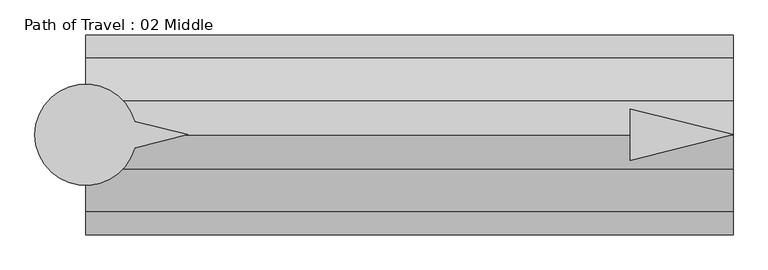
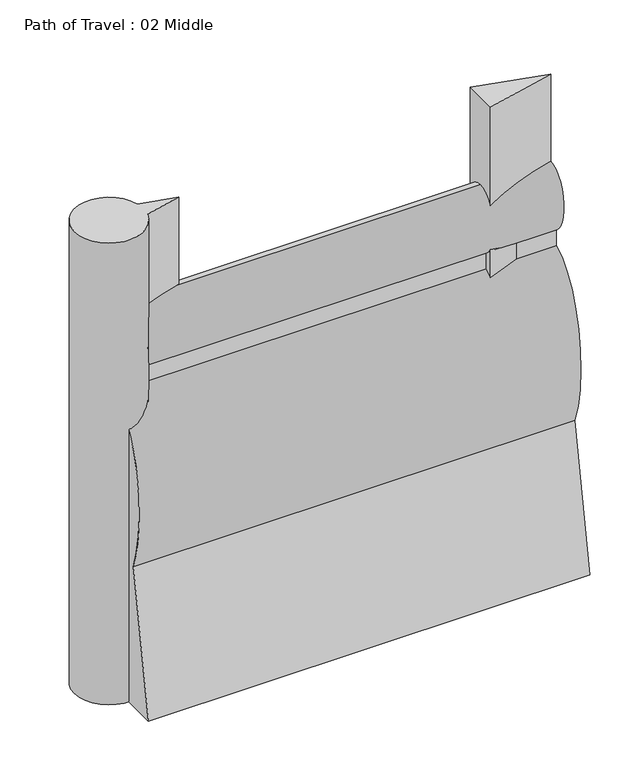
"""IFC4 building model written with IfcOpenShell, lengths in millimetres: proxy geometry, Path of Travel : 02 Middle."""

import ifcopenshell
import ifcopenshell.guid

model = None  # the IFC model being written
_history = None  # IfcOwnerHistory: only IFC2X3 demands one
_inside = {}  # id of a spatial element -> (the spatial element, [elements in it])
_under = {}  # id of a project, library or spatial element -> (it, [spatial elements below it])
_declared = {}  # id of a project -> (the project, [libraries it declares])
_typed = {}  # id of a type object -> (the type object, [elements of that type])
_made_of = {}  # id of a material, layer set ... -> (it, [elements and type objects made of it])


def new_model(schema):
    """Start an empty IFC model of exactly this schema.

    Asked for "IFC4X3", IfcOpenShell would pick the latest addendum, in which some entities
    have other attributes; the version numbers below select the first issue.
    IFC2X3 requires an IfcOwnerHistory on every rooted entity: one is made here for all.
    """
    global model, _history
    if schema == "IFC4X3":
        model = ifcopenshell.file(schema_version=(4, 3, 0, 0))
    else:
        model = ifcopenshell.file(schema=schema)
    _inside.clear()
    _under.clear()
    _declared.clear()
    _typed.clear()
    _made_of.clear()
    _history = None
    if model.schema == "IFC2X3":
        org = make("IfcOrganization", Name="unknown")
        user = make(
            "IfcPersonAndOrganization",
            ThePerson=make("IfcPerson", FamilyName="unknown"),
            TheOrganization=org,
        )
        app = make(
            "IfcApplication",
            ApplicationDeveloper=org,
            Version="unknown",
            ApplicationFullName="unknown",
            ApplicationIdentifier="unknown",
        )
        _history = make(
            "IfcOwnerHistory",
            OwningUser=user,
            OwningApplication=app,
            ChangeAction="ADDED",
            CreationDate=0,
        )
    return model


def make(cls, **values):
    """One entity of the class cls with the attributes given. An attribute that is None is left unset."""
    return model.create_entity(
        cls, **{name: value for name, value in values.items() if value is not None}
    )


def rooted(cls, **values):
    """An entity with a GlobalId (a new one), such as an element, a storey or a relation."""
    return make(cls, GlobalId=ifcopenshell.guid.new(), OwnerHistory=_history, **values)


def si_unit(unit_type, name, prefix=None):
    """IfcSIUnit, for example si_unit("LENGTHUNIT", "METRE", prefix="MILLI")."""
    return make("IfcSIUnit", UnitType=unit_type, Prefix=prefix, Name=name)


def assignment(units):
    """IfcUnitAssignment: the units of a project."""
    return None if units is None else make("IfcUnitAssignment", Units=units)


def point(xyz):
    """IfcCartesianPoint."""
    return None if xyz is None else make("IfcCartesianPoint", Coordinates=xyz)


def direction(xyz):
    """IfcDirection."""
    return None if xyz is None else make("IfcDirection", DirectionRatios=xyz)


def frame(location, z_axis=None, x_axis=None):
    """IfcAxis2Placement3D, a coordinate frame: its origin and axes. An axis left out is left unset."""
    return make(
        "IfcAxis2Placement3D",
        Location=point(location),
        Axis=direction(z_axis),
        RefDirection=direction(x_axis),
    )


def frame_2d(location, x_axis=None):
    """IfcAxis2Placement2D, a coordinate frame in the plane: its origin and x axis."""
    return make(
        "IfcAxis2Placement2D", Location=point(location), RefDirection=direction(x_axis)
    )


def origin():
    """The frame at (0, 0, 0) with its axes left unset."""
    return frame((0.0, 0.0, 0.0))


def origin_with_axes():
    """The frame at (0, 0, 0) with the z axis (0, 0, 1) and the x axis (1, 0, 0) written out."""
    return frame((0.0, 0.0, 0.0), z_axis=(0.0, 0.0, 1.0), x_axis=(1.0, 0.0, 0.0))


def place(relative_to, where):
    """IfcLocalPlacement: puts the frame where relative to a parent placement (None: the world)."""
    return make(
        "IfcLocalPlacement", PlacementRelTo=relative_to, RelativePlacement=where
    )


def context(
    kind, dimensions, precision=None, world=None, true_north=None, identifier=None
):
    """IfcGeometricRepresentationContext, for example the 3D "Model" context."""
    return make(
        "IfcGeometricRepresentationContext",
        ContextIdentifier=identifier,
        ContextType=kind,
        CoordinateSpaceDimension=dimensions,
        Precision=precision,
        WorldCoordinateSystem=world,
        TrueNorth=true_north,
    )


def project(units=None, contexts=None):
    """IfcProject with its units and contexts."""
    return rooted(
        "IfcProject",
        Name="project",
        RepresentationContexts=contexts,
        UnitsInContext=assignment(units),
    )


def spatial(cls, under=None, at=None, **own):
    """A site, building, storey or space (cls), placed at a placement, below another one or the project."""
    s = rooted(cls, ObjectPlacement=at, **own)
    if under is not None:
        _under.setdefault(under.id(), (under, []))[1].append(s)
    return s


def polyline(points):
    """IfcPolyline through the points."""
    return make("IfcPolyline", Points=[point(p) for p in points])


def circle_curve(where, radius):
    """IfcCircle in the frame where."""
    return make("IfcCircle", Position=where, Radius=radius)


def ellipse_curve(where, semi_axis1, semi_axis2):
    """IfcEllipse in the frame where."""
    return make(
        "IfcEllipse", Position=where, SemiAxis1=semi_axis1, SemiAxis2=semi_axis2
    )


def trimmed(basis, trim1, trim2, sense, master):
    """IfcTrimmedCurve: the piece of a basis curve between two trims."""
    return make(
        "IfcTrimmedCurve",
        BasisCurve=basis,
        Trim1=trim1,
        Trim2=trim2,
        SenseAgreement=sense,
        MasterRepresentation=master,
    )


def segment(curve, same_sense, transition):
    """IfcCompositeCurveSegment."""
    return make(
        "IfcCompositeCurveSegment",
        Transition=transition,
        SameSense=same_sense,
        ParentCurve=curve,
    )


def composite_curve(segments, self_intersect=None):
    """IfcCompositeCurve: segments joined end to end."""
    return make("IfcCompositeCurve", Segments=segments, SelfIntersect=self_intersect)


def outline(outer, holes=None, kind="AREA"):
    """IfcArbitraryClosedProfileDef: a profile drawn as a closed curve; with holes, ...WithVoids."""
    if holes is None:
        return make("IfcArbitraryClosedProfileDef", ProfileType=kind, OuterCurve=outer)
    return make(
        "IfcArbitraryProfileDefWithVoids",
        ProfileType=kind,
        OuterCurve=outer,
        InnerCurves=holes,
    )


def extrude(swept, where, along, depth):
    """IfcExtrudedAreaSolid: the profile swept, set in the frame where, extruded along a direction by depth."""
    return make(
        "IfcExtrudedAreaSolid",
        SweptArea=swept,
        Position=where,
        ExtrudedDirection=direction(along),
        Depth=depth,
    )


def shape(context_of_items, identifier, shape_type, items):
    """IfcShapeRepresentation: the items that make up one representation, for example the "Body"."""
    return make(
        "IfcShapeRepresentation",
        ContextOfItems=context_of_items,
        RepresentationIdentifier=identifier,
        RepresentationType=shape_type,
        Items=items,
    )


def source(mapping_origin, context_of_items, identifier, shape_type, items):
    """IfcRepresentationMap: a shape defined once, which mapped items show again and again."""
    return make(
        "IfcRepresentationMap",
        MappingOrigin=mapping_origin,
        MappedRepresentation=shape(context_of_items, identifier, shape_type, items),
    )


def transform(
    local_origin,
    x_axis=None,
    y_axis=None,
    z_axis=None,
    scale=None,
    scale2=None,
    scale3=None,
    uniform=True,
):
    """IfcCartesianTransformationOperator3D, or its non-uniform kind. x_axis, y_axis, z_axis: its Axis1, 2, 3."""
    if uniform:
        return make(
            "IfcCartesianTransformationOperator3D",
            Axis1=direction(x_axis),
            Axis2=direction(y_axis),
            LocalOrigin=point(local_origin),
            Scale=scale,
            Axis3=direction(z_axis),
        )
    return make(
        "IfcCartesianTransformationOperator3DnonUniform",
        Axis1=direction(x_axis),
        Axis2=direction(y_axis),
        LocalOrigin=point(local_origin),
        Scale=scale,
        Axis3=direction(z_axis),
        Scale2=scale2,
        Scale3=scale3,
    )


def mapped(mapping_source, mapping_target):
    """IfcMappedItem: shows the shape of a source again, moved by a transform."""
    return make(
        "IfcMappedItem", MappingSource=mapping_source, MappingTarget=mapping_target
    )


def made_of(thing, what):
    """Note that an element or type object is made of a material, layer set ...; save() writes the relation."""
    if what is not None:
        _made_of.setdefault(what.id(), (what, []))[1].append(thing)
    return thing


def element(
    cls,
    number,
    at=None,
    inside=None,
    cuts=None,
    type_object=None,
    material=None,
    context=None,
    identifier="Body",
    shape_type=None,
    held_by="IfcProductDefinitionShape",
    body=None,
    shapes=None,
    **own,
):
    """One element of the class cls, such as IfcWall. Its Tag is "e" and its number.

    at: its placement. inside: the storey or other place that contains it. cuts: it is an
    opening in that element (IfcRelVoidsElement). A single representation is given by context,
    identifier, shape_type and body (its items); several are given by shapes. held_by: the class
    of the entity that holds the representations. save() writes the other relations.
    """
    e = rooted(cls, Tag="e%d" % number, ObjectPlacement=at, **own)
    if body is not None:
        shapes = [shape(context, identifier, shape_type, body)]
    if shapes is not None:
        e.Representation = make(held_by, Representations=shapes)
    if inside is not None:
        _inside.setdefault(inside.id(), (inside, []))[1].append(e)
    if cuts is not None:
        rooted(
            "IfcRelVoidsElement", RelatingBuildingElement=cuts, RelatedOpeningElement=e
        )
    if type_object is not None:
        _typed.setdefault(type_object.id(), (type_object, []))[1].append(e)
    return made_of(e, material)


def aggregate(whole, parts):
    """IfcRelAggregates: a whole, such as a stair, and the parts it consists of."""
    return rooted("IfcRelAggregates", RelatingObject=whole, RelatedObjects=parts)


def save(model, path):
    """Write the relations noted so far, then the file.

    IfcRelAggregates (storeys below a building ...), IfcRelContainedInSpatialStructure (elements
    in a storey), IfcRelDefinesByType, IfcRelAssociatesMaterial and IfcRelDeclares: one each for
    every whole, place, type object, material and project.
    """
    for whole, parts in _under.values():
        aggregate(whole, parts)
    for where, things in _inside.values():
        rooted(
            "IfcRelContainedInSpatialStructure",
            RelatedElements=things,
            RelatingStructure=where,
        )
    for kind, things in _typed.values():
        rooted("IfcRelDefinesByType", RelatedObjects=things, RelatingType=kind)
    for what, things in _made_of.values():
        rooted("IfcRelAssociatesMaterial", RelatedObjects=things, RelatingMaterial=what)
    for by, libraries in _declared.values():
        rooted("IfcRelDeclares", RelatingContext=by, RelatedDefinitions=libraries)
    model.write(path)


def plane_surface(at):
    """IfcPlane: the flat surface through the origin of the frame at, square to its z axis."""
    return make("IfcPlane", Position=at)


def extruded_surface(curve, direction_of_extrusion, depth):
    """IfcSurfaceOfLinearExtrusion: the curve pushed along a direction by depth."""
    return make(
        "IfcSurfaceOfLinearExtrusion",
        SweptCurve=make("IfcArbitraryOpenProfileDef", ProfileType="CURVE", Curve=curve),
        ExtrudedDirection=direction(direction_of_extrusion),
        Depth=depth,
    )


def advanced_brep(points, edges, surfaces, faces):
    """IfcAdvancedBrep: a solid bounded by faces that lie on surfaces and meet in shared edges.

    An edge is (start, end): straight between two places in points (the first is 0);
    or (start, end, curve); or (start, end, curve, False) where it runs against its curve.
    A face is (place in surfaces, loops), or (place, loops, False) where it looks against
    its surface's normal. A loop lists edges by number (the first is 1), with a minus sign
    where the edge is run from its end to its start. The first loop is the outer one.
    """
    corners = [point(p) for p in points]
    vertices = [make("IfcVertexPoint", VertexGeometry=c) for c in corners]
    made = []
    for start, end, *more in edges:
        made.append(
            make(
                "IfcEdgeCurve",
                EdgeStart=vertices[start],
                EdgeEnd=vertices[end],
                EdgeGeometry=more[0] if more else make("IfcPolyline", Points=[corners[start], corners[end]]),
                SameSense=more[1] if len(more) > 1 else True,
            )
        )
    hull = []
    for where, loops, *sense in faces:
        bounds = []
        for j, loop in enumerate(loops):
            ring = [make("IfcOrientedEdge", EdgeElement=made[abs(k) - 1], Orientation=k > 0) for k in loop]
            bounds.append(
                make(
                    "IfcFaceOuterBound" if j == 0 else "IfcFaceBound",
                    Bound=make("IfcEdgeLoop", EdgeList=ring),
                    Orientation=True,
                )
            )
        hull.append(make("IfcAdvancedFace", Bounds=bounds, FaceSurface=surfaces[where], SameSense=sense[0] if sense else True))
    return make("IfcAdvancedBrep", Outer=make("IfcClosedShell", CfsFaces=hull))


def path_of_travel_02_middle_3647c35c(model_context):
    return source(origin(), model_context, "Body", "SolidModel", [
        advanced_brep(
        [(227.5554837, 0.0, 1727.2), (227.5554837, 42.9018657, 1436.6534209), (227.5554837, 42.9018657, 1363.4763406), (227.5554837, 184.1186263, 643.4144547), (227.5554837, 297.5699544, 0.0), (227.5554837, 145.6574193, 0.0), (227.5554837, 0.0, 584.2), (227.5554837, -145.6574193, 0.0), (227.5554837, -297.5699544, 0.0), (227.5554837, -184.1186263, 643.4144547), (227.5554837, -42.9018657, 1363.4763406), (227.5554837, -42.9018657, 1436.6534209), (2152.1530954, 0.0, 1727.2), (2152.1530954, -42.9018657, 1436.6534209), (2152.1530954, -42.9018657, 1363.4763406), (2152.1530954, -184.1186263, 643.4144547), (2152.1530954, -297.5699544, 0.0), (2152.1530954, -145.6574193, 0.0), (2152.1530954, 0.0, 584.2), (2152.1530954, 145.6574193, 0.0), (2152.1530954, 297.5699544, 0.0), (2152.1530954, 184.1186263, 643.4144547), (2152.1530954, 42.9018657, 1363.4763406), (2152.1530954, 42.9018657, 1436.6534209)],
        [
            (0, 1, ellipse_curve(frame((227.5554837, 0.0, 1574.8), z_axis=(-1.0, 0.0, 0.0), x_axis=(0.0, 0.0, 1.0)), 152.4, 101.6)),
            (1, 2),
            (2, 3, ellipse_curve(frame((227.5554837, 0.0, 914.4), z_axis=(-1.0, 0.0, 0.0), x_axis=(0.0, 0.0, -1.0)), 457.2, 228.6)),
            (3, 4),
            (4, 5),
            (5, 6),
            (6, 7),
            (7, 8),
            (8, 9),
            (9, 10, ellipse_curve(frame((227.5554837, 0.0, 914.4), z_axis=(-1.0, 0.0, 0.0), x_axis=(0.0, 0.0, -1.0)), 457.2, 228.6)),
            (10, 11),
            (11, 0, ellipse_curve(frame((227.5554837, 0.0, 1574.8), z_axis=(-1.0, 0.0, 0.0), x_axis=(0.0, 0.0, 1.0)), 152.4, 101.6)),
            (12, 13, ellipse_curve(frame((2152.1530954, 0.0, 1574.8), z_axis=(1.0, 0.0, 0.0), x_axis=(0.0, 0.0, 1.0)), 152.4, 101.6)),
            (13, 14),
            (14, 15, ellipse_curve(frame((2152.1530954, 0.0, 914.4), z_axis=(1.0, 0.0, 0.0), x_axis=(0.0, 0.0, -1.0)), 457.2, 228.6)),
            (15, 16),
            (16, 17),
            (17, 18),
            (18, 19),
            (19, 20),
            (20, 21),
            (21, 22, ellipse_curve(frame((2152.1530954, 0.0, 914.4), z_axis=(1.0, 0.0, 0.0), x_axis=(0.0, 0.0, -1.0)), 457.2, 228.6)),
            (22, 23),
            (23, 12, ellipse_curve(frame((2152.1530954, 0.0, 1574.8), z_axis=(1.0, 0.0, 0.0), x_axis=(0.0, 0.0, 1.0)), 152.4, 101.6)),
            (0, 12),
            (23, 1),
            (22, 2),
            (21, 3),
            (20, 4),
            (19, 5),
            (18, 6),
            (17, 7),
            (16, 8),
            (15, 9),
            (14, 10),
            (13, 11),
        ],
        [
            plane_surface(frame((227.5554837, 0.0, 0.0), z_axis=(-1.0, 0.0, 0.0), x_axis=(0.0, 0.0, 1.0))),
            plane_surface(frame((2152.1530954, 0.0, 0.0), z_axis=(1.0, 0.0, 0.0), x_axis=(0.0, 0.0, 1.0))),
            extruded_surface(trimmed(ellipse_curve(frame((2152.1530954, 0.0, 1574.8), z_axis=(-1.0, 0.0, 0.0), x_axis=(0.0, 0.0, 1.0)), 152.4, 101.6), [point((2152.1530954, 0.0, 1727.2))], [point((2152.1530954, 42.9018657, 1436.6534209))], True, "CARTESIAN"), (-1924.5976117, 0.0, 0.0), 1924.5976117),
            plane_surface(frame((227.5554837, 42.9018657, 1436.6534209), z_axis=(0.0, 1.0, 0.0), x_axis=(1.0, 0.0, 0.0))),
            extruded_surface(trimmed(ellipse_curve(frame((2152.1530954, 0.0, 914.4), z_axis=(-1.0, 0.0, 0.0), x_axis=(0.0, 0.0, -1.0)), 457.2, 228.6), [point((2152.1530954, 42.9018657, 1363.4763406))], [point((2152.1530954, 184.1186263, 643.4144547))], True, "CARTESIAN"), (-1924.5976117, 0.0, 0.0), 1924.5976117),
            plane_surface(frame((227.5554837, 184.1186263, 643.4144547), z_axis=(0.0, 0.9848077530122078, 0.1736481776669322), x_axis=(1.0, 0.0, 0.0))),
            plane_surface(frame((227.5554837, 297.5699544, 0.0), z_axis=(0.0, 0.0, -1.0), x_axis=(1.0, 0.0, 0.0))),
            plane_surface(frame((227.5554837, 145.6574193, 0.0), z_axis=(0.0, -0.9702957262760199, -0.2419218955995739), x_axis=(1.0, 0.0, 0.0))),
            plane_surface(frame((227.5554837, 0.0, 584.2), z_axis=(0.0, 0.9702957262759961, -0.24192189559966923), x_axis=(1.0, 0.0, 0.0))),
            plane_surface(frame((227.5554837, -145.6574193, 0.0), z_axis=(0.0, 0.0, -1.0), x_axis=(1.0, 0.0, 0.0))),
            plane_surface(frame((227.5554837, -297.5699544, 0.0), z_axis=(0.0, -0.984807753012208, 0.17364817766693066), x_axis=(1.0, 0.0, 0.0))),
            extruded_surface(trimmed(ellipse_curve(frame((2152.1530954, 0.0, 914.4), z_axis=(-1.0, 0.0, 0.0), x_axis=(0.0, 0.0, -1.0)), 457.2, 228.6), [point((2152.1530954, -184.1186263, 643.4144547))], [point((2152.1530954, -42.9018657, 1363.4763406))], True, "CARTESIAN"), (-1924.5976117, 0.0, 0.0), 1924.5976117),
            plane_surface(frame((227.5554837, -42.9018657, 1363.4763406), z_axis=(0.0, -1.0, 0.0), x_axis=(1.0, 0.0, 0.0))),
            extruded_surface(trimmed(ellipse_curve(frame((2152.1530954, 0.0, 1574.8), z_axis=(-1.0, 0.0, 0.0), x_axis=(0.0, 0.0, 1.0)), 152.4, 101.6), [point((2152.1530954, -42.9018657, 1436.6534209))], [point((2152.1530954, 0.0, 1727.2))], True, "CARTESIAN"), (-1924.5976117, 0.0, 0.0), 1924.5976117),
        ],
        [
            (0, [[1, 2, 3, 4, 5, 6, 7, 8, 9, 10, 11, 12]]),
            (1, [[13, 14, 15, 16, 17, 18, 19, 20, 21, 22, 23, 24]]),
            (2, [[-1, 25, -24, 26]]),
            (3, [[-2, -26, -23, 27]]),
            (4, [[-3, -27, -22, 28]]),
            (5, [[-4, -28, -21, 29]]),
            (6, [[-5, -29, -20, 30]]),
            (7, [[-6, -30, -19, 31]]),
            (8, [[-7, -31, -18, 32]]),
            (9, [[-8, -32, -17, 33]]),
            (10, [[-9, -33, -16, 34]]),
            (11, [[-10, -34, -15, 35]]),
            (12, [[-11, -35, -14, 36]]),
            (13, [[-12, -36, -13, -25]]),
        ],
    ),
        extrude(outline(polyline([(1846.1479489, 76.2006338), (2152.1530954, 0.0), (1846.1479489, -76.2006338), (1846.1479489, 76.2006338)])), origin_with_axes(), (0.0, 0.0, 1.0), 2129.5973753),
        extrude(outline(composite_curve([segment(polyline([(372.7837828, 39.4440225), (531.182385, 0.0), (372.7837828, -39.4440225)]), True, "CONTINUOUS"), segment(trimmed(circle_curve(frame_2d((227.2200886, 0.0)), 150.8131956), [point((372.7837828, -39.4440225))], [point((372.7837828, 39.4440225))], False, "CARTESIAN"), True, "CONTINUOUS")], self_intersect=False)), origin_with_axes(), (0.0, 0.0, 1.0), 2129.5973753),
    ])


if __name__ == "__main__":
    model = new_model("IFC4")
    model_context = context("Model", 3, world=origin())
    ifc_project = project(units=[si_unit("LENGTHUNIT", "METRE", prefix="MILLI")], contexts=[model_context])
    site = spatial("IfcSite", under=ifc_project)
    building = spatial("IfcBuilding", under=site)
    placement = place(None, origin())
    path_of_travel_02_middle_shape = path_of_travel_02_middle_3647c35c(model_context)
    element("IfcBuildingElementProxy", 1, Name="Path of Travel : 02 Middle", ObjectType="Path of Travel : 02 Middle", at=placement, inside=building, context=model_context, shape_type="MappedRepresentation", body=[
        mapped(path_of_travel_02_middle_shape, transform((0.0, 0.0, 0.0), x_axis=(1.0, 0.0, 0.0), y_axis=(0.0, 1.0, 0.0), z_axis=(0.0, 0.0, 1.0))),
    ])
    save(model, "model.ifc")

# Revit data of these elements
# Type "Path of Travel : 02 Middle"
#   Path of Egress [instance default] = 4' - 0"
#   built-in parameter 1001306 [instance default] = 4 (stored number, unit not read)
#   Dot at Start = no
#   Arrow in Middle = yes
#   Arrow at End = no
#   Egress Path = none
# Element 1 (IfcBuildingElementProxy, "Path of Travel : 02 Middle")
#   Path of Egress = 6' - 3.77156"
#   built-in parameter 1001306 = 6.3143 (stored number, unit not read)
#   Materials on its faces: "Egress Path Solid", "solid"
# Materials
#   "Egress Path Solid": class "Unassigned", colour RGB 255 128 64, transparency 0.75, Comments = "Rendering appearance not upgraded "
#   "solid": class "Generic", colour RGB 120 120 120, transparency 0, Cost = 0
